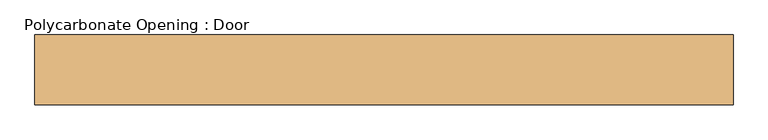
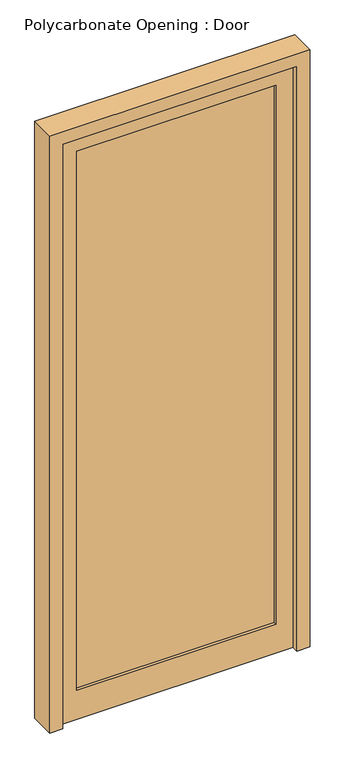
"""IFC4 building model written with IfcOpenShell, lengths in millimetres: door geometry, Polycarbonate Opening : Door."""

from ifc_helpers import new_model, si_unit, frame, origin, place, context, project, spatial, polyline, outline, extrude, source, transform, mapped, element, save


def polycarbonate_opening_door_552f9ae5(model_context):
    return source(origin(), model_context, "Body", "SweptSolid", [
        extrude(outline(polyline([(457.2, 0.0), (457.2, -25.4), (-457.2, -25.4), (-457.2, 0.0), (457.2, 0.0)])), frame((0.0, 0.0, 50.8), z_axis=(0.0, 0.0, 1.0), x_axis=(1.0, 0.0, 0.0)), (0.0, 0.0, 1.0), 2360.0132885),
        extrude(outline(polyline([(2410.8132885, -457.2), (0.0, -457.2), (0.0, 457.2), (2410.8132885, 457.2), (2410.8132885, -457.2)]), holes=[polyline([(119.0625, 388.9375), (119.0625, -388.9375), (2342.5507885, -388.9375), (2342.5507885, 388.9375), (119.0625, 388.9375)])]), frame((0.0, -38.1, 0.0), z_axis=(0.0, 1.0, 0.0), x_axis=(0.0, 0.0, 1.0)), (0.0, 0.0, 1.0), 50.8),
        extrude(outline(polyline([(2461.6132885, 508.0), (2461.6132885, -508.0), (0.0, -508.0), (0.0, -457.2), (2410.8132885, -457.2), (2410.8132885, 457.2), (0.0, 457.2), (0.0, 508.0), (2461.6132885, 508.0)])), frame((0.0, -63.5, 0.0), z_axis=(0.0, 1.0, 0.0), x_axis=(0.0, 0.0, 1.0)), (0.0, 0.0, 1.0), 101.6),
    ])


if __name__ == "__main__":
    model = new_model("IFC4")
    model_context = context("Model", 3, world=origin())
    ifc_project = project(units=[si_unit("LENGTHUNIT", "METRE", prefix="MILLI")], contexts=[model_context])
    site = spatial("IfcSite", under=ifc_project)
    building = spatial("IfcBuilding", under=site)
    placement = place(None, origin())
    polycarbonate_opening_door_shape = polycarbonate_opening_door_552f9ae5(model_context)
    element("IfcDoor", 1, ObjectType="Polycarbonate Opening : Door", at=placement, inside=building, context=model_context, shape_type="MappedRepresentation", body=[
        mapped(polycarbonate_opening_door_shape, transform((0.0, 0.0, 0.0), x_axis=(1.0, 0.0, 0.0), y_axis=(0.0, 1.0, 0.0), z_axis=(0.0, 0.0, 1.0))),
    ])
    save(model, "model.ifc")

# Revit data of these elements
# Type "Polycarbonate Opening : Door"
#   Type Mark = "60"
#   OD_DS_Door_Material = "ALUM./GLAZING"
#   OD_DS_Door_Type = "STOREFRONT (NARROW STILE)"
#   OD_DS_Lockset = "ENTRY LOCK (INSIDE ADA LEVER ALWAYS ACTIVE)"
#   Analytic Construction = "<None>"
#   offset [instance default] = 0' - 0 1/2"
#   Stile = 0' - 2 11/16"
#   Mullion Width = 0' - 2"
#   Mullion Depth = 0' - 4"
#   Opening Size [instance default] = 5' - 1.50212"
#   Door Width [instance default] = 5' - 1.50212"
#   Window ON/OFF = yes
#   Door On/Off = no
#   Mullion Material = KAWNEER 260 INSULCLADTM THERMAL ENTRANCE - CLEAR ANODIZED ALUM.
#   Glass Material = TEMPERED INSULATED GLAZING (CARDINAL GLASS LoĒ²-240\nOR EQUIVALENT)
#   Door Material = KAWNEER 260 INSULCLADTM THERMAL ENTRANCE - CLEAR ANODIZED ALUM.
# Element 1 (IfcDoor, "Polycarbonate Opening : Door")
#   Materials on its faces: "KAWNEER 260 INSULCLADTM THERMAL ENTRANCE - CLEAR ANODIZED ALUM.", "TEMPERED INSULATED GLAZING (CARDINAL GLASS LoĒ²-240\nOR EQUIVALENT)"
# Materials
#   "KAWNEER 260 INSULCLADTM THERMAL ENTRANCE - CLEAR ANODIZED ALUM.": class "Metal", colour RGB 244 244 244, transparency 0, Description = "Aluminum 6061", Cost = 0
#   "TEMPERED INSULATED GLAZING (CARDINAL GLASS LoĒ²-240\nOR EQUIVALENT)": class "Glass", colour RGB 196 205 210, transparency 0.85, Description = "Soda Lime Glass", Cost = 0
